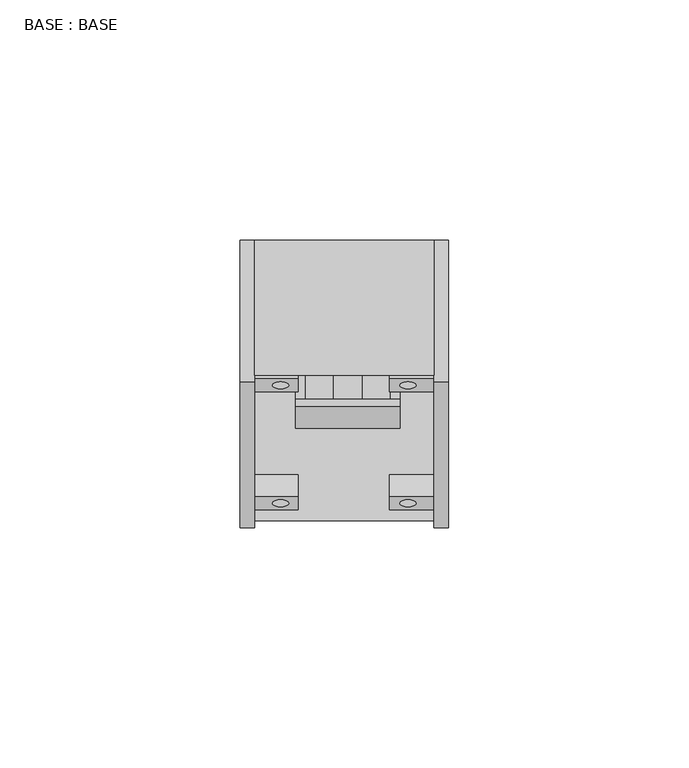
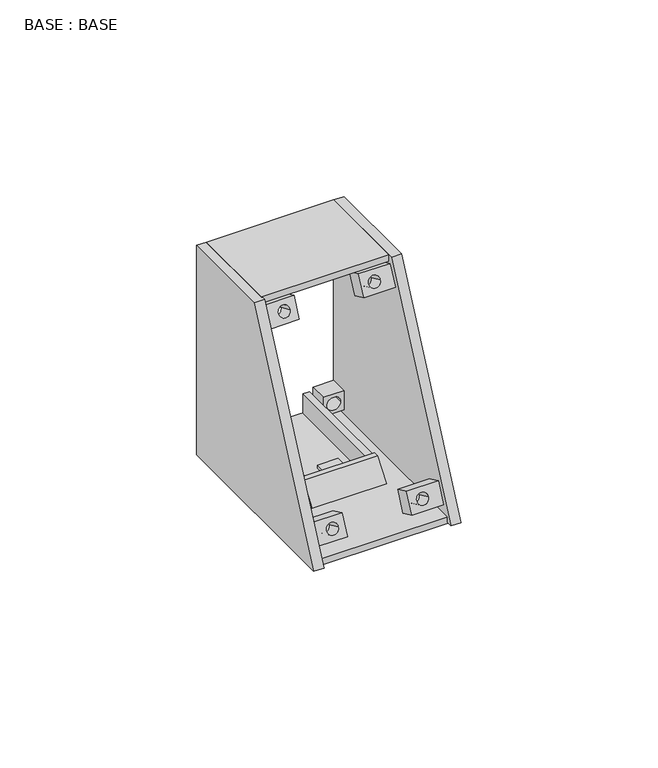
"""IFC4 building model written with IfcOpenShell, lengths in millimetres: proxy geometry, BASE : BASE."""

from ifc_helpers import new_model, si_unit, point, frame, frame_2d, origin, origin_with_axes, place, context, project, spatial, polyline, circle_curve, trimmed, segment, composite_curve, outline, extrude, source, transform, mapped, element, save


def base_base_f135f830(model_context):
    return source(origin(), model_context, "Body", "SweptSolid", [
        extrude(outline(polyline([(3.2, -2.2), (-3.2, -2.2), (-3.2, 7.1), (3.2, 7.1), (3.2, -2.2)]), holes=[composite_curve([segment(trimmed(circle_curve(frame_2d((0.0, 1.7)), 1.7), [point((0.0, 0.0))], [point((0.0, 3.4))], True, "CARTESIAN"), True, "CONTINUOUS"), segment(trimmed(circle_curve(frame_2d((0.0, 1.7)), 1.7), [point((0.0, 3.4))], [point((0.0, 0.0))], True, "CARTESIAN"), True, "CONTINUOUS")], self_intersect=False)]), frame((2402.2719295, 1326.1385366, 57.7208133), z_axis=(0.0, -0.9063077870366535, 0.4226182617406919), x_axis=(0.0, -0.4226182617406919, -0.9063077870366535)), (0.0, 0.0, 1.0), 5.0),
        extrude(outline(polyline([(3.2, -30.2), (-3.2, -30.2), (-3.2, -21.2), (3.2, -21.2), (3.2, -30.2)]), holes=[composite_curve([segment(trimmed(circle_curve(frame_2d((0.0, -24.8)), 1.7), [point((0.0, -23.1))], [point((0.0, -26.5))], True, "CARTESIAN"), True, "CONTINUOUS"), segment(trimmed(circle_curve(frame_2d((0.0, -24.8)), 1.7), [point((0.0, -26.5))], [point((0.0, -23.1))], True, "CARTESIAN"), True, "CONTINUOUS")], self_intersect=False)]), frame((2402.2719295, 1326.1385366, 57.7208133), z_axis=(0.0, -0.9063077870366535, 0.4226182617406919), x_axis=(0.0, -0.4226182617406919, -0.9063077870366535)), (0.0, 0.0, 1.0), 5.0),
        extrude(outline(polyline([(61.2, -2.2), (54.8, -2.2), (54.8, 7.1), (61.2, 7.1), (61.2, -2.2)]), holes=[composite_curve([segment(trimmed(circle_curve(frame_2d((58.0000001, 1.7)), 1.7), [point((58.0000001, 3.4))], [point((58.0000001, 0.0))], True, "CARTESIAN"), True, "CONTINUOUS"), segment(trimmed(circle_curve(frame_2d((58.0000001, 1.7)), 1.7), [point((58.0000001, 0.0))], [point((58.0000001, 3.4))], True, "CARTESIAN"), True, "CONTINUOUS")], self_intersect=False)]), frame((2402.2719295, 1326.1385366, 57.7208133), z_axis=(0.0, -0.9063077870366535, 0.4226182617406919), x_axis=(0.0, -0.4226182617406919, -0.9063077870366535)), (0.0, 0.0, 1.0), 5.0),
        extrude(outline(polyline([(61.2, -21.2), (61.2, -30.2), (54.8, -30.2), (54.8, -21.2), (61.2, -21.2)]), holes=[composite_curve([segment(trimmed(circle_curve(frame_2d((58.0000001, -24.8)), 1.7), [point((58.0000001, -23.1))], [point((58.0000001, -26.5))], True, "CARTESIAN"), True, "CONTINUOUS"), segment(trimmed(circle_curve(frame_2d((58.0000001, -24.8)), 1.7), [point((58.0000001, -26.5))], [point((58.0000001, -23.1))], True, "CARTESIAN"), True, "CONTINUOUS")], self_intersect=False)]), frame((2402.2719295, 1326.1385366, 57.7208133), z_axis=(0.0, -0.9063077870366535, 0.4226182617406919), x_axis=(0.0, -0.4226182617406919, -0.9063077870366535)), (0.0, 0.0, 1.0), 5.0),
        extrude(outline(polyline([(2394.4431854, 1318.7384159), (2388.4431854, 1318.7384159), (2388.4431854, 1323.7384159), (2394.4431854, 1323.7384159), (2394.4431854, 1318.7384159)])), frame((0.0, 0.0, 6.0), z_axis=(0.0, 0.0, 1.0), x_axis=(1.0, 0.0, 0.0)), (0.0, 0.0, 1.0), 1.0),
        extrude(outline(polyline([(1336.0781618, 2.0), (1344.7384159, 17.0), (1351.7384159, 17.0), (1351.7384159, 15.25), (1346.4884159, 15.25), (1346.4884159, 2.0), (1336.0781618, 2.0)])), frame((2372.0719295, 0.0, 0.0), z_axis=(1.0, 0.0, 0.0), x_axis=(0.0, 1.0, 0.0)), (0.0, 0.0, 1.0), 6.0),
        extrude(outline(polyline([(2409.3719295, 1323.7384159), (2372.0719295, 1323.7384159), (2372.0719295, 1351.7384159), (2409.3719295, 1351.7384159), (2409.3719295, 1323.7384159)])), frame((0.0, 0.0, 63.0), z_axis=(0.0, 0.0, 1.0), x_axis=(1.0, 0.0, 0.0)), (0.0, 0.0, 1.0), 2.0),
        extrude(outline(polyline([(3.0, 2403.3719295), (3.0, 2409.3719295), (9.0, 2409.3719295), (9.0, 2403.3719295), (3.0, 2403.3719295)]), holes=[composite_curve([segment(trimmed(circle_curve(frame_2d((6.0, 2406.3719295)), 2.0), [point((6.0, 2408.3719295))], [point((6.0, 2404.3719295))], True, "CARTESIAN"), True, "CONTINUOUS"), segment(trimmed(circle_curve(frame_2d((6.0, 2406.3719295)), 2.0), [point((6.0, 2404.3719295))], [point((6.0, 2408.3719295))], True, "CARTESIAN"), True, "CONTINUOUS")], self_intersect=False)]), frame((0.0, 1346.4884159, 0.0), z_axis=(0.0, 1.0, 0.0), x_axis=(0.0, 0.0, 1.0)), (0.0, 0.0, 1.0), 5.25),
        extrude(outline(polyline([(3.0, 2378.0719295), (9.0, 2378.0719295), (9.0, 2372.0719295), (3.0, 2372.0719295), (3.0, 2378.0719295)]), holes=[composite_curve([segment(trimmed(circle_curve(frame_2d((6.0, 2375.0719295)), 2.0), [point((6.0, 2377.0719295))], [point((6.0, 2373.0719295))], True, "CARTESIAN"), True, "CONTINUOUS"), segment(trimmed(circle_curve(frame_2d((6.0, 2375.0719295)), 2.0), [point((6.0, 2373.0719295))], [point((6.0, 2377.0719295))], True, "CARTESIAN"), True, "CONTINUOUS")], self_intersect=False)]), frame((0.0, 1346.4884159, 0.0), z_axis=(0.0, 1.0, 0.0), x_axis=(0.0, 0.0, 1.0)), (0.0, 0.0, 1.0), 5.25),
        extrude(outline(polyline([(62.0, 2403.3719295), (56.0, 2403.3719295), (56.0, 2409.3719295), (62.0, 2409.3719295), (62.0, 2403.3719295)]), holes=[composite_curve([segment(trimmed(circle_curve(frame_2d((59.0, 2406.3719295)), 2.0), [point((59.0, 2408.3719295))], [point((59.0, 2404.3719295))], True, "CARTESIAN"), True, "CONTINUOUS"), segment(trimmed(circle_curve(frame_2d((59.0, 2406.3719295)), 2.0), [point((59.0, 2404.3719295))], [point((59.0, 2408.3719295))], True, "CARTESIAN"), True, "CONTINUOUS")], self_intersect=False)]), frame((0.0, 1346.4884159, 0.0), z_axis=(0.0, 1.0, 0.0), x_axis=(0.0, 0.0, 1.0)), (0.0, 0.0, 1.0), 5.25),
        extrude(outline(polyline([(62.0, 2378.0719295), (62.0, 2372.0719295), (56.0, 2372.0719295), (56.0, 2378.0719295), (62.0, 2378.0719295)]), holes=[composite_curve([segment(trimmed(circle_curve(frame_2d((59.0, 2375.0719295)), 2.0), [point((59.0, 2377.0719295))], [point((59.0, 2373.0719295))], True, "CARTESIAN"), True, "CONTINUOUS"), segment(trimmed(circle_curve(frame_2d((59.0, 2375.0719295)), 2.0), [point((59.0, 2373.0719295))], [point((59.0, 2377.0719295))], True, "CARTESIAN"), True, "CONTINUOUS")], self_intersect=False)]), frame((0.0, 1346.4884159, 0.0), z_axis=(0.0, 1.0, 0.0), x_axis=(0.0, 0.0, 1.0)), (0.0, 0.0, 1.0), 5.25),
        extrude(outline(polyline([(1351.7384159, 0.0), (1292.0509228, 0.0), (1322.3609206, 65.0), (1351.7384159, 65.0), (1351.7384159, 0.0)])), frame((2409.3719295, 0.0, 0.0), z_axis=(1.0, 0.0, 0.0), x_axis=(0.0, 1.0, 0.0)), (0.0, 0.0, 1.0), 3.0),
        extrude(outline(polyline([(1351.7384159, 0.0), (1292.0509228, 0.0), (1322.3609206, 65.0), (1351.7384159, 65.0), (1351.7384159, 0.0)])), frame((2369.0719295, 0.0, 0.0), z_axis=(1.0, 0.0, 0.0), x_axis=(0.0, 1.0, 0.0)), (0.0, 0.0, 1.0), 3.0),
        extrude(outline(polyline([(2402.3331854, 1318.7384159), (2400.3331854, 1318.7384159), (2400.3331854, 1351.7384159), (2402.3331854, 1351.7384159), (2402.3331854, 1318.7384159)])), frame((0.0, 0.0, 2.0), z_axis=(0.0, 0.0, 1.0), x_axis=(1.0, 0.0, 0.0)), (0.0, 0.0, 1.0), 6.0),
        extrude(outline(polyline([(2380.5531854, 1318.7384159), (2380.5531854, 1351.7384159), (2382.5531854, 1351.7384159), (2382.5531854, 1318.7384159), (2380.5531854, 1318.7384159)])), frame((0.0, 0.0, 2.0), z_axis=(0.0, 0.0, 1.0), x_axis=(1.0, 0.0, 0.0)), (0.0, 0.0, 1.0), 6.0),
        extrude(outline(polyline([(1318.7384159, 9.0), (1318.7384159, 3.0), (1312.7384159, 3.0), (1317.2253325, 9.0), (1318.7384159, 9.0)])), frame((2380.5531854, 0.0, 0.0), z_axis=(1.0, 0.0, 0.0), x_axis=(0.0, 1.0, 0.0)), (0.0, 0.0, 1.0), 21.78),
        extrude(outline(polyline([(2409.3719295, 1293.4498458), (2372.0719295, 1293.4498458), (2372.0719295, 1351.7384159), (2409.3719295, 1351.7384159), (2409.3719295, 1293.4498458)])), origin_with_axes(), (0.0, 0.0, 1.0), 2.0),
    ])


if __name__ == "__main__":
    model = new_model("IFC4")
    model_context = context("Model", 3, world=origin())
    ifc_project = project(units=[si_unit("LENGTHUNIT", "METRE", prefix="MILLI")], contexts=[model_context])
    site = spatial("IfcSite", under=ifc_project)
    building = spatial("IfcBuilding", under=site)
    placement = place(None, origin())
    base_base_shape = base_base_f135f830(model_context)
    element("IfcBuildingElementProxy", 1, Name="BASE : BASE", ObjectType="BASE : BASE", at=placement, inside=building, context=model_context, shape_type="MappedRepresentation", body=[
        mapped(base_base_shape, transform((0.0, 0.0, 0.0), x_axis=(1.0, 0.0, 0.0), y_axis=(0.0, 1.0, 0.0), z_axis=(0.0, 0.0, 1.0))),
    ])
    save(model, "model.ifc")

# Revit data of these elements
# Project information
#   Data de emissão do projeto = "Data de emissão"
#   Status do projeto = "Status do projeto"
#   Nome do cliente = "Proprietário"
#   Endereço do projeto = "Insira aqui o endereço"
#   Nome do projeto = "Nome do projeto"
#   Número do projeto = "0001"
# Element 1 (IfcBuildingElementProxy, "BASE : BASE")
#   Materials on its faces: ".BOX LATERAL"
# Materials
#   ".BOX LATERAL": class "Vidro", colour RGB 236 240 239, transparency 0.15, Cost = 0
